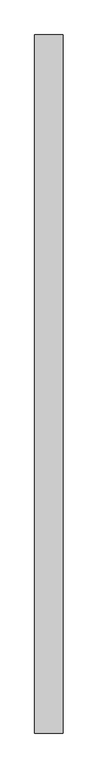
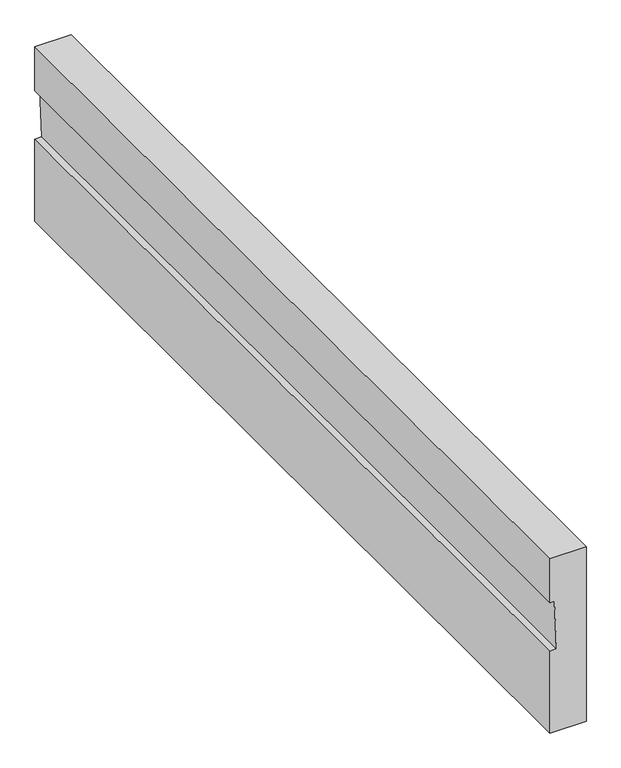
"""IFC4 building model written with IfcOpenShell, lengths in millimetres: proxy geometry, Generic Models 7:Generic Models 1:1:Generic Models 1:1 : Generic Models 7:Generic Models 1:337419:41 : Generic Models 7:Generic Models 1:1:Generic Models 1:1 : Generic Models 7:Generic Models 1:337419:306201."""

from ifc_helpers import new_model, si_unit, origin, place, context, project, spatial, faceted_brep, source, transform, mapped, element, save


def generic_models_3486df04(model_context):
    return source(origin(), model_context, "Body", "Brep", [
        faceted_brep([(579107.289849, -573942.9163841, 4983.1625), (579304.933599, -573942.9163841, 4983.1625), (579304.933599, -573942.9163841, 4077.2484422), (579247.1208806, -573942.9163841, 4077.2484422), (579247.1208806, -573942.9163841, 3981.4775028), (579107.289849, -573942.9163841, 3981.4775028), (579107.289849, -573942.9163841, 4451.1570938), (579143.9316077, -573942.9163841, 4452.6838337), (579132.3000335, -573942.9163841, 4731.8416143), (579107.289849, -573942.9163841, 4730.7995233), (579107.289849, -578797.4913841, 3981.4775028), (579304.933599, -578797.4913841, 3981.4775028), (579304.933599, -578797.4913841, 4983.1625), (579107.289849, -578797.4913841, 4983.1625), (579107.289849, -578797.4913841, 4730.7995233), (579132.3000335, -578797.4913841, 4731.8416143), (579143.9316077, -578797.4913841, 4452.6838337), (579107.289849, -578797.4913841, 4451.1570938), (579304.933599, -577227.6325678, 3981.4775028), (579304.933599, -573944.6255932, 4118.2694601), (579247.1208806, -577227.6325678, 3981.4775028), (579247.1208806, -573944.6255932, 4118.2694601)], [[[0, 1, 2, 3, 4, 5, 6, 7, 8, 9]], [[10, 11, 12, 13, 14, 15, 16, 17]], [[1, 0, 13, 12]], [[12, 11, 18, 19, 2, 1]], [[11, 10, 5, 4, 20, 18]], [[13, 0, 9, 14]], [[15, 14, 9, 8]], [[16, 15, 8, 7]], [[5, 10, 17, 6]], [[16, 7, 6, 17]], [[19, 21, 3, 2]], [[3, 21, 20, 4]], [[21, 19, 18, 20]]]),
    ])


if __name__ == "__main__":
    model = new_model("IFC4")
    model_context = context("Model", 3, world=origin())
    ifc_project = project(units=[si_unit("LENGTHUNIT", "METRE", prefix="MILLI")], contexts=[model_context])
    site = spatial("IfcSite", under=ifc_project)
    building = spatial("IfcBuilding", under=site)
    placement = place(None, origin())
    generic_models_shape = generic_models_3486df04(model_context)
    element("IfcBuildingElementProxy", 1, Name="Generic Models 7:Generic Models 1:1:Generic Models 1:1 : Generic Models 7:Generic Models 1:337419:41 : Generic Models 7:Generic Models 1:1:Generic Models 1:1 : Generic Models 7:Generic Models 1:337419:306201", ObjectType="Generic Models 7:Generic Models 1:1:Generic Models 1:1 : Generic Models 7:Generic Models 1:337419:41 : Generic Models 7:Generic Models 1:1:Generic Models 1:1 : Generic Models 7:Generic Models 1:337419:306201", at=placement, inside=building, context=model_context, shape_type="MappedRepresentation", body=[
        mapped(generic_models_shape, transform((0.0, 0.0, 0.0), x_axis=(1.0, 0.0, 0.0), y_axis=(0.0, 1.0, 0.0), z_axis=(0.0, 0.0, 1.0))),
    ])
    save(model, "model.ifc")

# Revit data of these elements
# Type "Generic Models 7:Generic Models 1:1:Generic Models 1:1 : Generic Models 7:Generic Models 1:337419:41 : Generic Models 7:Generic Models 1:1:Generic Models 1:1 : Generic Models 7:Generic Models 1:337419:306201"
#   NameOverride = "Generic Models 7:Generic Models 1:1:Generic Models 1:1 : Generic Models 7:Generic Models 1:337419:306201"
#   ObjectTypeOverride = "Generic Models 1:1 : Generic Models 7:Generic Models 1:337419"
#   Reference = "Generic Models 1"
#   Tag = "306201"
# Element 1 (IfcBuildingElementProxy, "Generic Models 7:Generic Models 1:1:Generic Models 1:1 : Generic Models 7:Generic Models 1:337419:41 : Generic Models 7:Generic Models 1:1:Generic Models 1:1 : Generic Models 7:Generic Models 1:337419:306201")
#   Materials on its faces: "FULL CAVITY CLASS A FIBERGLASS INSULATION WITH DURABLE VAPOR BARRIER (BLACK) LINER"
# Materials
#   "FULL CAVITY CLASS A FIBERGLASS INSULATION WITH DURABLE VAPOR BARRIER (BLACK) LINER": class "Unassigned", colour RGB 158 92 175, transparency 0, Cost = 0
